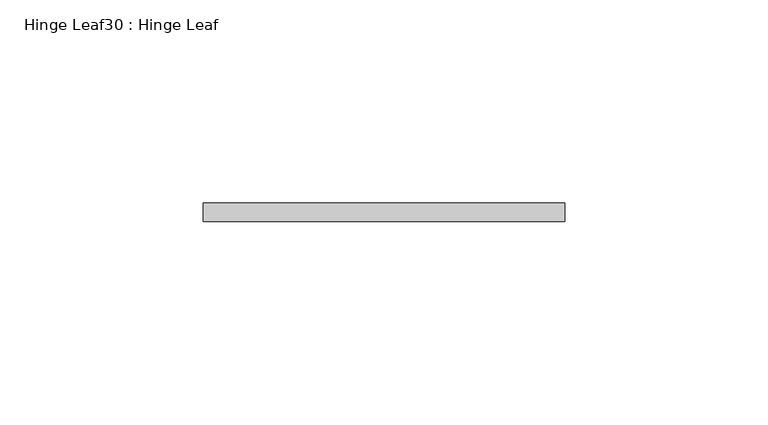
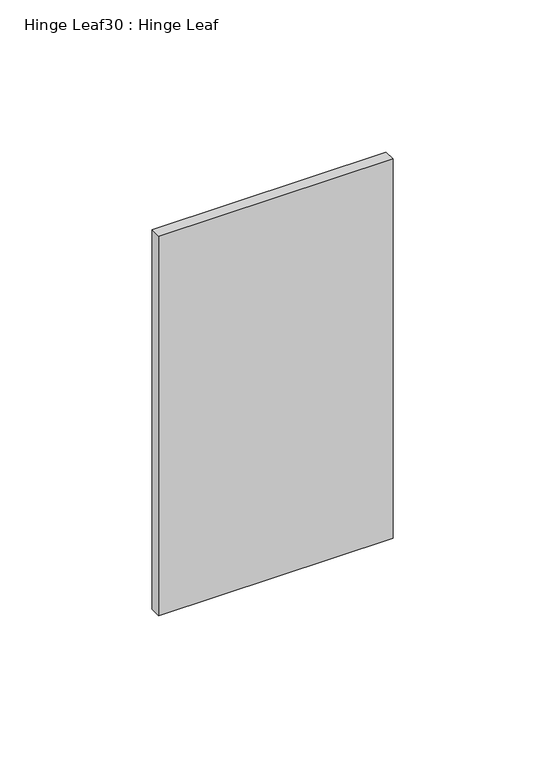
"""IFC4 building model written with IfcOpenShell, lengths in millimetres: proxy geometry, Hinge Leaf30 : Hinge Leaf."""

import ifcopenshell
import ifcopenshell.guid

model = None  # the IFC model being written
_history = None  # IfcOwnerHistory: only IFC2X3 demands one
_inside = {}  # id of a spatial element -> (the spatial element, [elements in it])
_under = {}  # id of a project, library or spatial element -> (it, [spatial elements below it])
_declared = {}  # id of a project -> (the project, [libraries it declares])
_typed = {}  # id of a type object -> (the type object, [elements of that type])
_made_of = {}  # id of a material, layer set ... -> (it, [elements and type objects made of it])


def new_model(schema):
    """Start an empty IFC model of exactly this schema.

    Asked for "IFC4X3", IfcOpenShell would pick the latest addendum, in which some entities
    have other attributes; the version numbers below select the first issue.
    IFC2X3 requires an IfcOwnerHistory on every rooted entity: one is made here for all.
    """
    global model, _history
    if schema == "IFC4X3":
        model = ifcopenshell.file(schema_version=(4, 3, 0, 0))
    else:
        model = ifcopenshell.file(schema=schema)
    _inside.clear()
    _under.clear()
    _declared.clear()
    _typed.clear()
    _made_of.clear()
    _history = None
    if model.schema == "IFC2X3":
        org = make("IfcOrganization", Name="unknown")
        user = make(
            "IfcPersonAndOrganization",
            ThePerson=make("IfcPerson", FamilyName="unknown"),
            TheOrganization=org,
        )
        app = make(
            "IfcApplication",
            ApplicationDeveloper=org,
            Version="unknown",
            ApplicationFullName="unknown",
            ApplicationIdentifier="unknown",
        )
        _history = make(
            "IfcOwnerHistory",
            OwningUser=user,
            OwningApplication=app,
            ChangeAction="ADDED",
            CreationDate=0,
        )
    return model


def make(cls, **values):
    """One entity of the class cls with the attributes given. An attribute that is None is left unset."""
    return model.create_entity(
        cls, **{name: value for name, value in values.items() if value is not None}
    )


def rooted(cls, **values):
    """An entity with a GlobalId (a new one), such as an element, a storey or a relation."""
    return make(cls, GlobalId=ifcopenshell.guid.new(), OwnerHistory=_history, **values)


def si_unit(unit_type, name, prefix=None):
    """IfcSIUnit, for example si_unit("LENGTHUNIT", "METRE", prefix="MILLI")."""
    return make("IfcSIUnit", UnitType=unit_type, Prefix=prefix, Name=name)


def assignment(units):
    """IfcUnitAssignment: the units of a project."""
    return None if units is None else make("IfcUnitAssignment", Units=units)


def point(xyz):
    """IfcCartesianPoint."""
    return None if xyz is None else make("IfcCartesianPoint", Coordinates=xyz)


def direction(xyz):
    """IfcDirection."""
    return None if xyz is None else make("IfcDirection", DirectionRatios=xyz)


def frame(location, z_axis=None, x_axis=None):
    """IfcAxis2Placement3D, a coordinate frame: its origin and axes. An axis left out is left unset."""
    return make(
        "IfcAxis2Placement3D",
        Location=point(location),
        Axis=direction(z_axis),
        RefDirection=direction(x_axis),
    )


def origin():
    """The frame at (0, 0, 0) with its axes left unset."""
    return frame((0.0, 0.0, 0.0))


def place(relative_to, where):
    """IfcLocalPlacement: puts the frame where relative to a parent placement (None: the world)."""
    return make(
        "IfcLocalPlacement", PlacementRelTo=relative_to, RelativePlacement=where
    )


def context(
    kind, dimensions, precision=None, world=None, true_north=None, identifier=None
):
    """IfcGeometricRepresentationContext, for example the 3D "Model" context."""
    return make(
        "IfcGeometricRepresentationContext",
        ContextIdentifier=identifier,
        ContextType=kind,
        CoordinateSpaceDimension=dimensions,
        Precision=precision,
        WorldCoordinateSystem=world,
        TrueNorth=true_north,
    )


def project(units=None, contexts=None):
    """IfcProject with its units and contexts."""
    return rooted(
        "IfcProject",
        Name="project",
        RepresentationContexts=contexts,
        UnitsInContext=assignment(units),
    )


def spatial(cls, under=None, at=None, **own):
    """A site, building, storey or space (cls), placed at a placement, below another one or the project."""
    s = rooted(cls, ObjectPlacement=at, **own)
    if under is not None:
        _under.setdefault(under.id(), (under, []))[1].append(s)
    return s


def polyline(points):
    """IfcPolyline through the points."""
    return make("IfcPolyline", Points=[point(p) for p in points])


def outline(outer, holes=None, kind="AREA"):
    """IfcArbitraryClosedProfileDef: a profile drawn as a closed curve; with holes, ...WithVoids."""
    if holes is None:
        return make("IfcArbitraryClosedProfileDef", ProfileType=kind, OuterCurve=outer)
    return make(
        "IfcArbitraryProfileDefWithVoids",
        ProfileType=kind,
        OuterCurve=outer,
        InnerCurves=holes,
    )


def extrude(swept, where, along, depth):
    """IfcExtrudedAreaSolid: the profile swept, set in the frame where, extruded along a direction by depth."""
    return make(
        "IfcExtrudedAreaSolid",
        SweptArea=swept,
        Position=where,
        ExtrudedDirection=direction(along),
        Depth=depth,
    )


def shape(context_of_items, identifier, shape_type, items):
    """IfcShapeRepresentation: the items that make up one representation, for example the "Body"."""
    return make(
        "IfcShapeRepresentation",
        ContextOfItems=context_of_items,
        RepresentationIdentifier=identifier,
        RepresentationType=shape_type,
        Items=items,
    )


def source(mapping_origin, context_of_items, identifier, shape_type, items):
    """IfcRepresentationMap: a shape defined once, which mapped items show again and again."""
    return make(
        "IfcRepresentationMap",
        MappingOrigin=mapping_origin,
        MappedRepresentation=shape(context_of_items, identifier, shape_type, items),
    )


def transform(
    local_origin,
    x_axis=None,
    y_axis=None,
    z_axis=None,
    scale=None,
    scale2=None,
    scale3=None,
    uniform=True,
):
    """IfcCartesianTransformationOperator3D, or its non-uniform kind. x_axis, y_axis, z_axis: its Axis1, 2, 3."""
    if uniform:
        return make(
            "IfcCartesianTransformationOperator3D",
            Axis1=direction(x_axis),
            Axis2=direction(y_axis),
            LocalOrigin=point(local_origin),
            Scale=scale,
            Axis3=direction(z_axis),
        )
    return make(
        "IfcCartesianTransformationOperator3DnonUniform",
        Axis1=direction(x_axis),
        Axis2=direction(y_axis),
        LocalOrigin=point(local_origin),
        Scale=scale,
        Axis3=direction(z_axis),
        Scale2=scale2,
        Scale3=scale3,
    )


def mapped(mapping_source, mapping_target):
    """IfcMappedItem: shows the shape of a source again, moved by a transform."""
    return make(
        "IfcMappedItem", MappingSource=mapping_source, MappingTarget=mapping_target
    )


def made_of(thing, what):
    """Note that an element or type object is made of a material, layer set ...; save() writes the relation."""
    if what is not None:
        _made_of.setdefault(what.id(), (what, []))[1].append(thing)
    return thing


def element(
    cls,
    number,
    at=None,
    inside=None,
    cuts=None,
    type_object=None,
    material=None,
    context=None,
    identifier="Body",
    shape_type=None,
    held_by="IfcProductDefinitionShape",
    body=None,
    shapes=None,
    **own,
):
    """One element of the class cls, such as IfcWall. Its Tag is "e" and its number.

    at: its placement. inside: the storey or other place that contains it. cuts: it is an
    opening in that element (IfcRelVoidsElement). A single representation is given by context,
    identifier, shape_type and body (its items); several are given by shapes. held_by: the class
    of the entity that holds the representations. save() writes the other relations.
    """
    e = rooted(cls, Tag="e%d" % number, ObjectPlacement=at, **own)
    if body is not None:
        shapes = [shape(context, identifier, shape_type, body)]
    if shapes is not None:
        e.Representation = make(held_by, Representations=shapes)
    if inside is not None:
        _inside.setdefault(inside.id(), (inside, []))[1].append(e)
    if cuts is not None:
        rooted(
            "IfcRelVoidsElement", RelatingBuildingElement=cuts, RelatedOpeningElement=e
        )
    if type_object is not None:
        _typed.setdefault(type_object.id(), (type_object, []))[1].append(e)
    return made_of(e, material)


def aggregate(whole, parts):
    """IfcRelAggregates: a whole, such as a stair, and the parts it consists of."""
    return rooted("IfcRelAggregates", RelatingObject=whole, RelatedObjects=parts)


def save(model, path):
    """Write the relations noted so far, then the file.

    IfcRelAggregates (storeys below a building ...), IfcRelContainedInSpatialStructure (elements
    in a storey), IfcRelDefinesByType, IfcRelAssociatesMaterial and IfcRelDeclares: one each for
    every whole, place, type object, material and project.
    """
    for whole, parts in _under.values():
        aggregate(whole, parts)
    for where, things in _inside.values():
        rooted(
            "IfcRelContainedInSpatialStructure",
            RelatedElements=things,
            RelatingStructure=where,
        )
    for kind, things in _typed.values():
        rooted("IfcRelDefinesByType", RelatedObjects=things, RelatingType=kind)
    for what, things in _made_of.values():
        rooted("IfcRelAssociatesMaterial", RelatedObjects=things, RelatingMaterial=what)
    for by, libraries in _declared.values():
        rooted("IfcRelDeclares", RelatingContext=by, RelatedDefinitions=libraries)
    model.write(path)


def hinge_leaf30_hinge_leaf_a1326aa5(model_context):
    return source(origin(), model_context, "Body", "SweptSolid", [
        extrude(outline(polyline([(587327.7934739, -531780.6943841), (587416.6934739, -531780.6943841), (587416.6934739, -531785.2663841), (587327.7934739, -531785.2663841), (587327.7934739, -531780.6943841)])), frame((0.0, 0.0, 1123.95), z_axis=(0.0, 0.0, 1.0), x_axis=(1.0, 0.0, 0.0)), (0.0, 0.0, 1.0), 152.4),
    ])


if __name__ == "__main__":
    model = new_model("IFC4")
    model_context = context("Model", 3, world=origin())
    ifc_project = project(units=[si_unit("LENGTHUNIT", "METRE", prefix="MILLI")], contexts=[model_context])
    site = spatial("IfcSite", under=ifc_project)
    building = spatial("IfcBuilding", under=site)
    placement = place(None, origin())
    hinge_leaf30_hinge_leaf_shape = hinge_leaf30_hinge_leaf_a1326aa5(model_context)
    element("IfcBuildingElementProxy", 1, Name="Hinge Leaf30 : Hinge Leaf", ObjectType="Hinge Leaf30 : Hinge Leaf", at=placement, inside=building, context=model_context, shape_type="MappedRepresentation", body=[
        mapped(hinge_leaf30_hinge_leaf_shape, transform((0.0, 0.0, 0.0), x_axis=(1.0, 0.0, 0.0), y_axis=(0.0, 1.0, 0.0), z_axis=(0.0, 0.0, 1.0))),
    ])
    save(model, "model.ifc")

# Revit data of these elements
# Element 1 (IfcBuildingElementProxy, "Hinge Leaf30 : Hinge Leaf")
#   Materials on its faces: "6\"X6\" WELD-ON STL BUTT HINGE"
# Materials
#   "6\"X6\" WELD-ON STL BUTT HINGE": class "Metal", colour RGB 189 187 185, transparency 0, Description = "Carbon steel", Cost = 0
